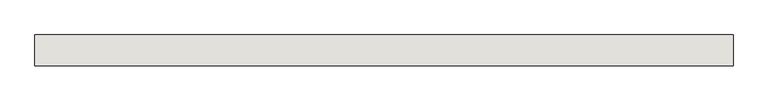
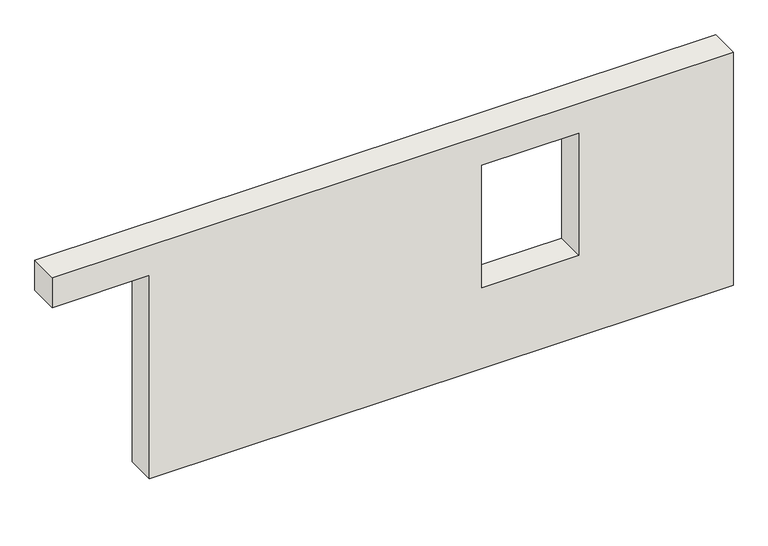
"""IFC4 building model written with IfcOpenShell, lengths in millimetres: wall geometry, 0_3d."""

from ifc_helpers import new_model, si_unit, frame, origin, place, context, project, spatial, polyline, outline, extrude, source, transform, mapped, element, save


def wall_dcefb690(model_context):
    return source(origin(), model_context, "Body", "SweptSolid", [
        extrude(outline(polyline([(2510.0, 0.0), (2510.0, 1135.0), (0.0, 1135.0), (0.0, 7950.0), (2880.0, 7950.0), (2880.0, 0.0), (2510.0, 0.0)]), holes=[polyline([(1000.0, 5015.0), (2510.0, 5015.0), (2510.0, 6150.0), (1000.0, 6150.0), (1000.0, 5015.0)])]), frame((0.0, 0.0, 0.0), z_axis=(0.0, 1.0, 0.0), x_axis=(0.0, 0.0, 1.0)), (0.0, 0.0, 1.0), 350.0),
    ])


if __name__ == "__main__":
    model = new_model("IFC4")
    model_context = context("Model", 3, world=origin())
    ifc_project = project(units=[si_unit("LENGTHUNIT", "METRE", prefix="MILLI")], contexts=[model_context])
    site = spatial("IfcSite", under=ifc_project)
    building = spatial("IfcBuilding", under=site)
    placement = place(None, origin())
    wall_shape = wall_dcefb690(model_context)
    element("IfcWall", 1, ObjectType="0_3d", at=placement, inside=building, context=model_context, shape_type="MappedRepresentation", body=[
        mapped(wall_shape, transform((0.0, 0.0, 0.0), x_axis=(1.0, 0.0, 0.0), y_axis=(0.0, 1.0, 0.0), z_axis=(0.0, 0.0, 1.0))),
    ])
    save(model, "model.ifc")

# Revit data of these elements
# Element 1 (IfcWall, "0_3d")
#   Materials on its faces: "holzschalung"
# Materials
#   "holzschalung": class "Unassigned", colour RGB 128 128 128, transparency 0
